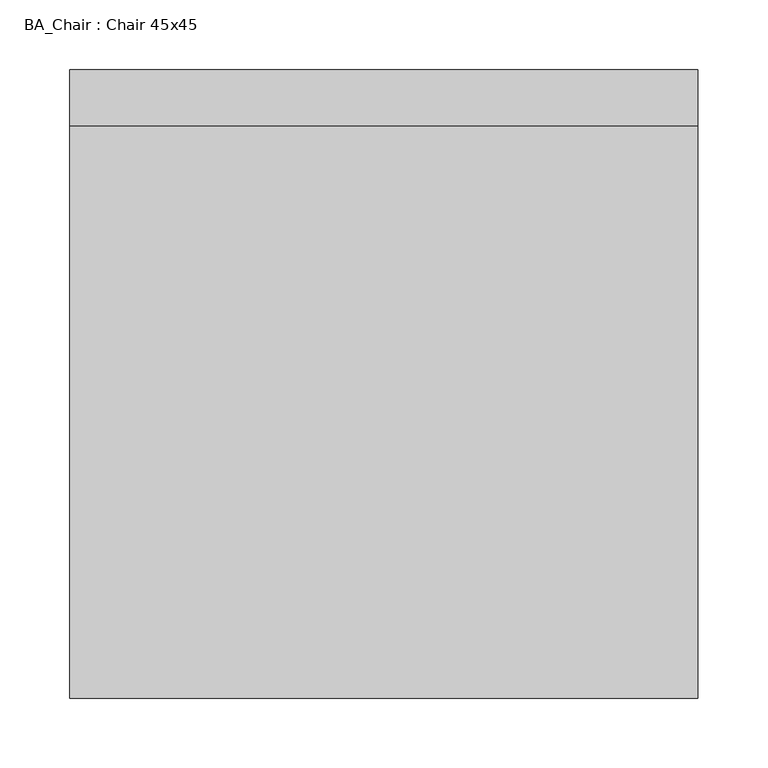
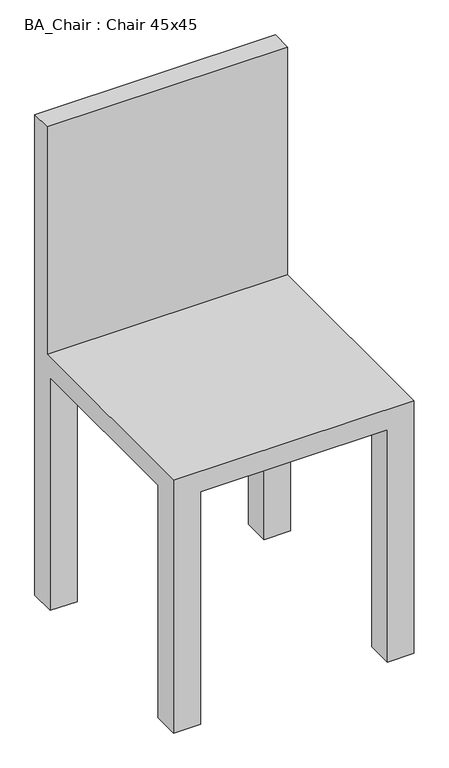
"""IFC4 building model written with IfcOpenShell, lengths in millimetres: furniture geometry, BA_Chair : Chair 45x45."""

from ifc_helpers import new_model, si_unit, origin, place, context, project, spatial, faceted_brep, source, transform, mapped, element, save


def ba_chair_chair_45x45_10945a81(model_context):
    return source(origin(), model_context, "Body", "Brep", [
        faceted_brep([(225.0, -225.0, 500.0), (225.0, -225.0, 0.0), (225.0, -175.0, 0.0), (225.0, -175.0, 460.0), (225.0, 175.0, 460.0), (225.0, 175.0, 0.0), (225.0, 225.0, 0.0), (225.0, 225.0, 950.0), (225.0, 185.0, 950.0), (225.0, 185.0, 500.0), (-225.0, 225.0, 950.0), (-225.0, 225.0, 0.0), (-225.0, 175.0, 0.0), (-225.0, 175.0, 460.0), (-225.0, -175.0, 460.0), (-225.0, -175.0, 0.0), (-225.0, -225.0, 0.0), (-225.0, -225.0, 500.0), (-225.0, 185.0, 500.0), (-225.0, 185.0, 950.0), (-175.0, 175.0, 460.0), (-175.0, 225.0, 460.0), (175.0, 225.0, 460.0), (175.0, 175.0, 460.0), (175.0, -175.0, 460.0), (175.0, -225.0, 460.0), (-175.0, -225.0, 460.0), (-175.0, -175.0, 460.0), (-175.0, -225.0, 0.0), (175.0, -225.0, 0.0), (175.0, 225.0, 0.0), (-175.0, 225.0, 0.0), (-175.0, 175.0, 0.0), (-175.0, -175.0, 0.0), (175.0, -175.0, 0.0), (175.0, 175.0, 0.0)], [[[0, 1, 2, 3, 4, 5, 6, 7, 8, 9]], [[10, 11, 12, 13, 14, 15, 16, 17, 18, 19]], [[20, 21, 22, 23, 4, 3, 24, 25, 26, 27, 14, 13]], [[17, 16, 28, 26, 25, 29, 1, 0]], [[9, 18, 17, 0]], [[8, 19, 18, 9]], [[7, 10, 19, 8]], [[6, 30, 22, 21, 31, 11, 10, 7]], [[32, 12, 11, 31]], [[32, 20, 13, 12]], [[31, 21, 20, 32]], [[28, 16, 15, 33]], [[15, 14, 27, 33]], [[33, 27, 26, 28]], [[1, 29, 34, 2]], [[29, 25, 24, 34]], [[34, 24, 3, 2]], [[5, 35, 30, 6]], [[5, 4, 23, 35]], [[35, 23, 22, 30]]]),
    ])


if __name__ == "__main__":
    model = new_model("IFC4")
    model_context = context("Model", 3, world=origin())
    ifc_project = project(units=[si_unit("LENGTHUNIT", "METRE", prefix="MILLI")], contexts=[model_context])
    site = spatial("IfcSite", under=ifc_project)
    building = spatial("IfcBuilding", under=site)
    placement = place(None, origin())
    ba_chair_chair_45x45_shape = ba_chair_chair_45x45_10945a81(model_context)
    element("IfcFurniture", 1, ObjectType="BA_Chair : Chair 45x45", at=placement, inside=building, context=model_context, shape_type="MappedRepresentation", body=[
        mapped(ba_chair_chair_45x45_shape, transform((0.0, 0.0, 0.0), x_axis=(1.0, 0.0, 0.0), y_axis=(0.0, 1.0, 0.0), z_axis=(0.0, 0.0, 1.0))),
    ])
    save(model, "model.ifc")

# Revit data of these elements
# Type "BA_Chair : Chair 45x45"
#   visina stolice = 500 mm
#   visina naslona = 450 mm
#   sirina/duzina stolice = 450 mm
#   Default Elevation = 0
# Element 1 (IfcFurniture, "BA_Chair : Chair 45x45")
#   Materials on its faces: "Default"
# Materials
#   "Default": class "Generic", colour RGB 255 255 255, transparency 0, Cost = 0
